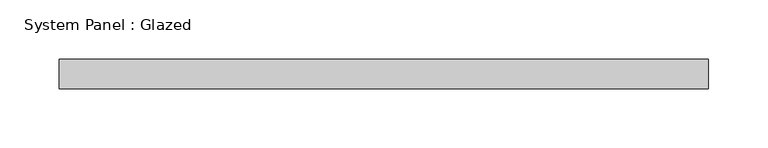
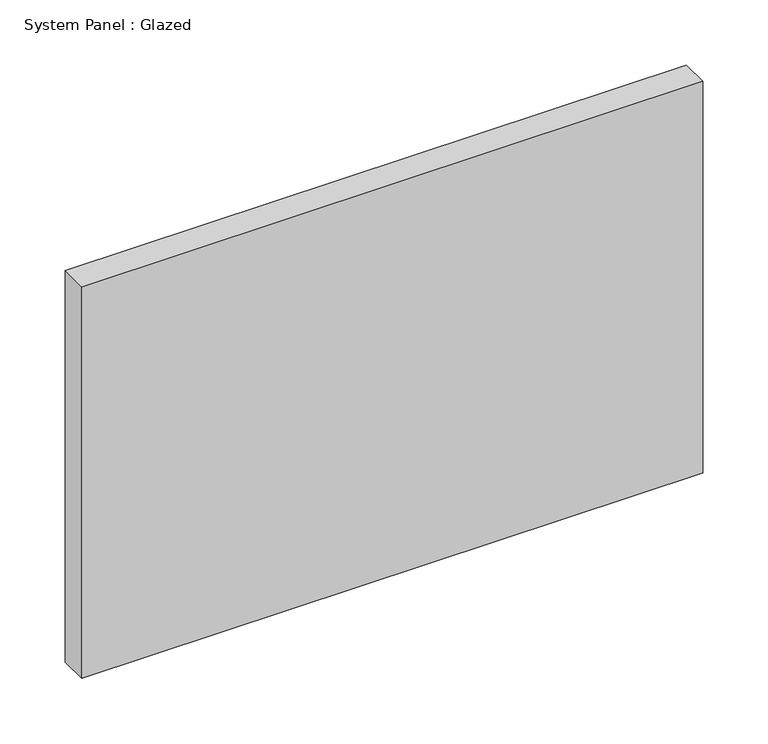
"""IFC4 building model written with IfcOpenShell, lengths in millimetres: plate geometry, System Panel : Glazed."""

from ifc_helpers import new_model, si_unit, origin, origin_with_axes, place, context, project, spatial, polyline, outline, extrude, source, transform, mapped, element, save


def system_panel_glazed_67b4cafa(model_context):
    return source(origin(), model_context, "Body", "SweptSolid", [
        extrude(outline(polyline([(275.0, 24.5), (-275.0, 24.5), (-275.0, 49.5), (275.0, 49.5), (275.0, 24.5)])), origin_with_axes(), (0.0, 0.0, 1.0), 366.6666667),
    ])


if __name__ == "__main__":
    model = new_model("IFC4")
    model_context = context("Model", 3, world=origin())
    ifc_project = project(units=[si_unit("LENGTHUNIT", "METRE", prefix="MILLI")], contexts=[model_context])
    site = spatial("IfcSite", under=ifc_project)
    building = spatial("IfcBuilding", under=site)
    placement = place(None, origin())
    system_panel_glazed_shape = system_panel_glazed_67b4cafa(model_context)
    element("IfcPlate", 1, ObjectType="System Panel : Glazed", at=placement, inside=building, context=model_context, shape_type="MappedRepresentation", body=[
        mapped(system_panel_glazed_shape, transform((0.0, 0.0, 0.0), x_axis=(1.0, 0.0, 0.0), y_axis=(0.0, 1.0, 0.0), z_axis=(0.0, 0.0, 1.0))),
    ])
    save(model, "model.ifc")

# Revit data of these elements
# Element 1 (IfcPlate, "System Panel : Glazed")
#   Materials on its faces: "Glass"
# Materials
#   "Glass": class "Glass", colour RGB 218 227 224, transparency 0.85, Description = "Soda Lime Glass", Cost = 0
